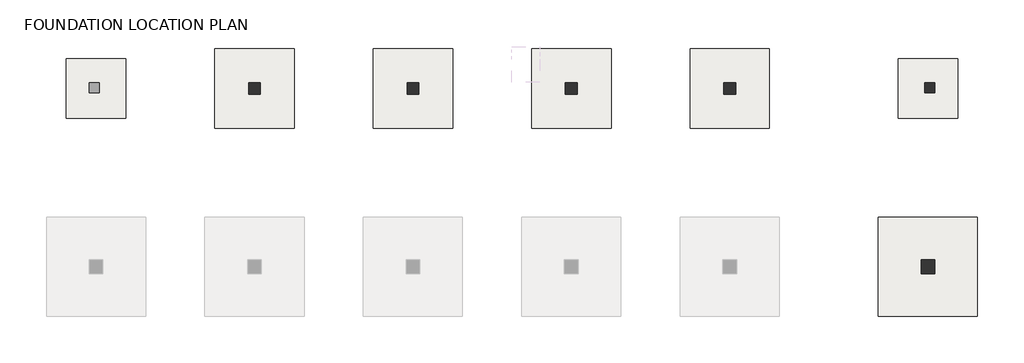
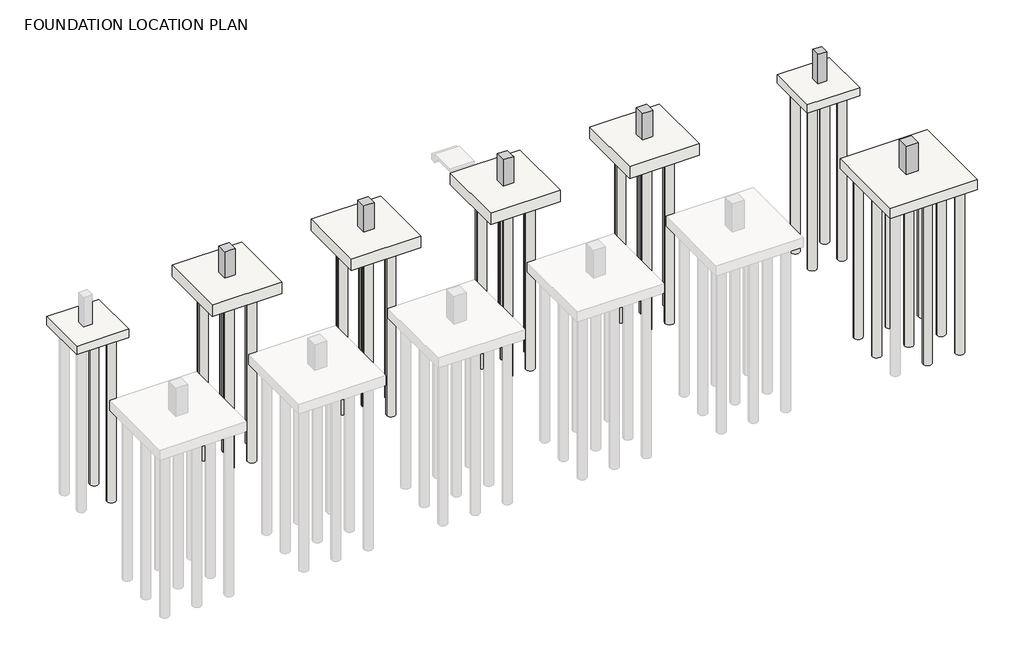
# One storey, part 3 of 3: 49 slabs, 6 columns.
"""IFC4 building model written with IfcOpenShell, lengths in millimetres."""

from ifc_helpers import new_model, si_unit, point, frame, frame_2d, origin, place, context, project, spatial, polyline, circle_curve, trimmed, segment, composite_curve, outline, extrude, faceted_brep, element, save

model = new_model("IFC4")

# Units and contexts
model_context = context("Model", 3, world=origin())
ifc_project = project(units=[si_unit("LENGTHUNIT", "METRE", prefix="MILLI")], contexts=[model_context])

# Site, building, storey
site = spatial("IfcSite", under=ifc_project)
building = spatial("IfcBuilding", under=site)
storey = spatial("IfcBuildingStorey", under=building, Name="FOUNDATION LOCATION PLAN", Elevation=-1699.994759)

# Columns
placement = place(None, origin())
element("IfcColumn", 1, ObjectType="Concrete-Rectangular-Column_R1 : CLS111_RC COLUMN_UG_C1", at=placement, inside=storey, context=model_context, shape_type="Brep", body=[
    faceted_brep([(41850.0, 39299.5208589, -1199.994759), (42350.0, 39299.5208589, -1199.994759), (42350.0, 38799.5208589, -1199.994759), (41850.0, 38799.5208589, -1199.994759), (41850.0, 39299.5208589, 600.005241), (42350.0, 39299.5208589, 600.005241), (41850.0, 38799.5208589, 450.005241), (41850.0, 38799.5208589, 600.005241), (41850.0, 38999.7368538, 600.005241), (42350.0, 38799.5208589, 600.005241), (42000.0, 38799.5208589, 600.005241)], [[[0, 1, 2, 3]], [[1, 0, 4, 5]], [[0, 3, 6, 7, 8, 4]], [[3, 2, 9, 10, 7, 6]], [[2, 1, 5, 9]], [[5, 4, 8, 7, 10, 9]]]),
])
element("IfcColumn", 2, ObjectType="Concrete-Rectangular-Column_R1 : CLS111_RC COLUMN_UG_C3", at=placement, inside=storey, context=model_context, shape_type="Brep", body=[
    faceted_brep([(41650.0, 30349.5208589, -1099.994759), (42350.0, 30349.5208589, -1099.994759), (42350.0, 29649.5208589, -1099.994759), (41650.0, 29649.5208589, -1099.994759), (41650.0, 30349.5208589, 450.005241), (41650.0, 30349.5208589, 600.005241), (42000.0, 30349.5208589, 600.005241), (42350.0, 30349.5208589, 600.005241), (41650.0, 29649.5208589, 450.005241), (41650.0, 29649.5208589, 600.005241), (42350.0, 29649.5208589, 600.005241)], [[[0, 1, 2, 3]], [[1, 0, 4, 5, 6, 7]], [[0, 3, 8, 9, 5, 4]], [[3, 2, 10, 9, 8]], [[2, 1, 7, 10]], [[5, 9, 10, 7, 6]]]),
])
element("IfcColumn", 3, ObjectType="Concrete-Rectangular-Column_R1 : CLS111_RC COLUMN_UG_C2", at=placement, inside=storey, context=model_context, shape_type="Brep", body=[
    faceted_brep([(7700.0, 39299.7368538, -999.994759), (8300.0, 39299.7368538, -999.994759), (8300.0, 38699.7368538, -999.994759), (7700.0, 38699.7368538, -999.994759), (7700.0, 39299.7368538, 600.005241), (8300.0, 39299.7368538, 600.005241), (8300.0, 39299.5208589, 600.005241), (8300.0, 38999.7634659, 600.005241), (8300.0, 38699.7368538, 600.005241), (8300.0, 38699.7368538, 450.005241), (8100.0, 38699.7368538, 600.005241), (7700.0, 38699.7368538, 600.005241), (7700.0, 38699.7368538, 450.005241), (7700.0, 38699.7368538, 0.005241), (7700.0, 38999.7368538, 600.005241), (7700.0, 39299.5208589, 600.005241)], [[[0, 1, 2, 3]], [[1, 0, 4, 5]], [[2, 1, 5, 6, 7, 8, 9]], [[3, 2, 9, 8, 10, 11, 12, 13]], [[0, 3, 13, 12, 11, 14, 15, 4]], [[5, 4, 15, 14, 11, 10, 8, 7, 6]]]),
])
element("IfcColumn", 4, ObjectType="Concrete-Rectangular-Column_R1 : CLS111_RC COLUMN_UG_C2", at=placement, inside=storey, context=model_context, shape_type="Brep", body=[
    faceted_brep([(15700.0, 39299.7368538, -999.994759), (16300.0, 39299.7368538, -999.994759), (16300.0, 38699.7368538, -999.994759), (15700.0, 38699.7368538, -999.994759), (15700.0, 39299.7368538, 600.005241), (16300.0, 39299.7368538, 600.005241), (16300.0, 39299.5208589, 600.005241), (16300.0, 38999.7368538, 600.005241), (16300.0, 38699.7368538, 600.005241), (16300.0, 38699.7368538, 450.005241), (16200.0, 38699.7368538, 600.005241), (15800.0, 38699.7368538, 600.005241), (15700.0, 38699.7368538, 600.005241), (15700.0, 38699.7368538, 450.005241), (15700.0, 38999.7634659, 600.005241), (15700.0, 39299.5208589, 600.005241)], [[[0, 1, 2, 3]], [[1, 0, 4, 5]], [[2, 1, 5, 6, 7, 8, 9]], [[3, 2, 9, 8, 10, 11, 12, 13]], [[0, 3, 13, 12, 14, 15, 4]], [[5, 4, 15, 14, 12, 11, 10, 8, 7, 6]]]),
])
element("IfcColumn", 5, ObjectType="Concrete-Rectangular-Column_R1 : CLS111_RC COLUMN_UG_C2", at=placement, inside=storey, context=model_context, shape_type="Brep", body=[
    faceted_brep([(23700.0, 39299.7368538, -999.994759), (24300.0, 39299.7368538, -999.994759), (24300.0, 38699.7368538, -999.994759), (23700.0, 38699.7368538, -999.994759), (23700.0, 39299.7368538, 600.005241), (24300.0, 39299.7368538, 600.005241), (24300.0, 39299.5208589, 600.005241), (24300.0, 38999.7368538, 600.005241), (24300.0, 38699.7368538, 600.005241), (24300.0, 38699.7368538, 450.005241), (24200.0, 38699.7368538, 600.005241), (23800.0, 38699.7368538, 600.005241), (23700.0, 38699.7368538, 600.005241), (23700.0, 38699.7368538, 450.005241), (23700.0, 38999.7368538, 600.005241), (23700.0, 39299.5208589, 600.005241)], [[[0, 1, 2, 3]], [[1, 0, 4, 5]], [[2, 1, 5, 6, 7, 8, 9]], [[3, 2, 9, 8, 10, 11, 12, 13]], [[0, 3, 13, 12, 14, 15, 4]], [[5, 4, 15, 14, 12, 11, 10, 8, 7, 6]]]),
])
element("IfcColumn", 6, ObjectType="Concrete-Rectangular-Column_R1 : CLS111_RC COLUMN_UG_C2", at=placement, inside=storey, context=model_context, shape_type="Brep", body=[
    faceted_brep([(31700.0, 39299.7368538, -999.994759), (32300.0, 39299.7368538, -999.994759), (32300.0, 38699.7368538, -999.994759), (31700.0, 38699.7368538, -999.994759), (31700.0, 39299.7368538, 600.005241), (32300.0, 39299.7368538, 600.005241), (32300.0, 39299.5208589, 600.005241), (32300.0, 38999.7368538, 600.005241), (32300.0, 38699.7368538, 600.005241), (32300.0, 38699.7368538, 450.005241), (32200.0, 38699.7368538, 600.005241), (31800.0, 38699.7368538, 600.005241), (31700.0, 38699.7368538, 600.005241), (31700.0, 38699.7368538, 450.005241), (31700.0, 38999.7368538, 600.005241), (31700.0, 39299.5208589, 600.005241)], [[[0, 1, 2, 3]], [[1, 0, 4, 5]], [[2, 1, 5, 6, 7, 8, 9]], [[3, 2, 9, 8, 10, 11, 12, 13]], [[0, 3, 13, 12, 14, 15, 4]], [[5, 4, 15, 14, 12, 11, 10, 8, 7, 6]]]),
])

# Slabs
element("IfcSlab", 7, ObjectType="Footing-Rectangular_R1 : FTS301_Footing-Rectangular_3000x3000x500_F1", at=placement, inside=storey, context=model_context, shape_type="SweptSolid", body=[
    extrude(outline(polyline([(1500.0, 40499.7368538), (1500.0, 37499.7368538), (-1500.0, 37499.7368538), (-1500.0, 40499.7368538), (1500.0, 40499.7368538)])), frame((0.0, 0.0, -1699.994759), z_axis=(0.0, 0.0, 1.0), x_axis=(1.0, 0.0, 0.0)), (0.0, 0.0, 1.0), 500.0),
])
element("IfcSlab", 8, ObjectType="Footing-Rectangular_R1 : FTS301_Footing-Rectangular_3000x3000x500_F1", at=placement, inside=storey, context=model_context, shape_type="SweptSolid", body=[
    extrude(outline(polyline([(43500.0, 40499.7368538), (43500.0, 37499.7368538), (40500.0, 37499.7368538), (40500.0, 40499.7368538), (43500.0, 40499.7368538)])), frame((0.0, 0.0, -1699.994759), z_axis=(0.0, 0.0, 1.0), x_axis=(1.0, 0.0, 0.0)), (0.0, 0.0, 1.0), 500.0),
])
element("IfcSlab", 9, ObjectType="Footing-Rectangular_R1 : FTS301_Footing-Rectangular_4000x4000x700_F2", at=placement, inside=storey, context=model_context, shape_type="SweptSolid", body=[
    extrude(outline(polyline([(10000.0, 40999.7368538), (10000.0, 36999.7368538), (6000.0, 36999.7368538), (6000.0, 40999.7368538), (10000.0, 40999.7368538)])), frame((0.0, 0.0, -1699.994759), z_axis=(0.0, 0.0, 1.0), x_axis=(1.0, 0.0, 0.0)), (0.0, 0.0, 1.0), 700.0),
])
element("IfcSlab", 10, ObjectType="Footing-Rectangular_R1 : FTS301_Footing-Rectangular_4000x4000x700_F2", at=placement, inside=storey, context=model_context, shape_type="SweptSolid", body=[
    extrude(outline(polyline([(18000.0, 40999.7368538), (18000.0, 36999.7368538), (14000.0, 36999.7368538), (14000.0, 40999.7368538), (18000.0, 40999.7368538)])), frame((0.0, 0.0, -1699.994759), z_axis=(0.0, 0.0, 1.0), x_axis=(1.0, 0.0, 0.0)), (0.0, 0.0, 1.0), 700.0),
])
element("IfcSlab", 11, ObjectType="Footing-Rectangular_R1 : FTS301_Footing-Rectangular_4000x4000x700_F2", at=placement, inside=storey, context=model_context, shape_type="SweptSolid", body=[
    extrude(outline(polyline([(26000.0, 40999.7368538), (26000.0, 36999.7368538), (22000.0, 36999.7368538), (22000.0, 40999.7368538), (26000.0, 40999.7368538)])), frame((0.0, 0.0, -1699.994759), z_axis=(0.0, 0.0, 1.0), x_axis=(1.0, 0.0, 0.0)), (0.0, 0.0, 1.0), 700.0),
])
element("IfcSlab", 12, ObjectType="Footing-Rectangular_R1 : FTS301_Footing-Rectangular_4000x4000x700_F2", at=placement, inside=storey, context=model_context, shape_type="SweptSolid", body=[
    extrude(outline(polyline([(34000.0, 40999.7368538), (34000.0, 36999.7368538), (30000.0, 36999.7368538), (30000.0, 40999.7368538), (34000.0, 40999.7368538)])), frame((0.0, 0.0, -1699.994759), z_axis=(0.0, 0.0, 1.0), x_axis=(1.0, 0.0, 0.0)), (0.0, 0.0, 1.0), 700.0),
])
element("IfcSlab", 13, ObjectType="Footing-Rectangular_R1 : FTS301_Footing-Rectangular_5000x5000x600_F3", at=placement, inside=storey, context=model_context, shape_type="SweptSolid", body=[
    extrude(outline(polyline([(44500.0, 32499.5208589), (44500.0, 27499.5208589), (39500.0, 27499.5208589), (39500.0, 32499.5208589), (44500.0, 32499.5208589)])), frame((0.0, 0.0, -1699.994759), z_axis=(0.0, 0.0, 1.0), x_axis=(1.0, 0.0, 0.0)), (0.0, 0.0, 1.0), 600.0),
])
element("IfcSlab", 14, ObjectType="HEC_PILE : FTPS102_D500", at=placement, inside=storey, context=model_context, shape_type="SweptSolid", body=[
    extrude(outline(composite_curve([segment(trimmed(circle_curve(frame_2d((850.0, 39849.5208589)), 250.0), [point((600.0, 39849.5208589))], [point((1100.0, 39849.5208589))], False, "CARTESIAN"), True, "CONTINUOUS"), segment(trimmed(circle_curve(frame_2d((850.0, 39849.5208589)), 250.0), [point((1100.0, 39849.5208589))], [point((600.0, 39849.5208589))], False, "CARTESIAN"), True, "CONTINUOUS")], self_intersect=False)), frame((0.0, 0.0, -11749.994759), z_axis=(0.0, 0.0, 1.0), x_axis=(1.0, 0.0, 0.0)), (0.0, 0.0, 1.0), 10150.0),
])
element("IfcSlab", 15, ObjectType="HEC_PILE : FTPS102_D500", at=placement, inside=storey, context=model_context, shape_type="SweptSolid", body=[
    extrude(outline(composite_curve([segment(trimmed(circle_curve(frame_2d((41150.0, 39849.5208589)), 250.0), [point((41400.0, 39849.5208589))], [point((40900.0, 39849.5208589))], False, "CARTESIAN"), True, "CONTINUOUS"), segment(trimmed(circle_curve(frame_2d((41150.0, 39849.5208589)), 250.0), [point((40900.0, 39849.5208589))], [point((41400.0, 39849.5208589))], False, "CARTESIAN"), True, "CONTINUOUS")], self_intersect=False)), frame((0.0, 0.0, -11749.994759), z_axis=(0.0, 0.0, 1.0), x_axis=(1.0, 0.0, 0.0)), (0.0, 0.0, 1.0), 10150.0),
])
element("IfcSlab", 16, ObjectType="HEC_PILE : FTPS102_D500", at=placement, inside=storey, context=model_context, shape_type="SweptSolid", body=[
    extrude(outline(composite_curve([segment(trimmed(circle_curve(frame_2d((42850.0, 39849.5208589)), 250.0), [point((42600.0, 39849.5208589))], [point((43100.0, 39849.5208589))], False, "CARTESIAN"), True, "CONTINUOUS"), segment(trimmed(circle_curve(frame_2d((42850.0, 39849.5208589)), 250.0), [point((43100.0, 39849.5208589))], [point((42600.0, 39849.5208589))], False, "CARTESIAN"), True, "CONTINUOUS")], self_intersect=False)), frame((0.0, 0.0, -11749.994759), z_axis=(0.0, 0.0, 1.0), x_axis=(1.0, 0.0, 0.0)), (0.0, 0.0, 1.0), 10150.0),
])
element("IfcSlab", 17, ObjectType="HEC_PILE : FTPS102_D500", at=placement, inside=storey, context=model_context, shape_type="SweptSolid", body=[
    extrude(outline(composite_curve([segment(trimmed(circle_curve(frame_2d((41150.0, 38149.5208589)), 250.0), [point((41400.0, 38149.5208589))], [point((40900.0, 38149.5208589))], False, "CARTESIAN"), True, "CONTINUOUS"), segment(trimmed(circle_curve(frame_2d((41150.0, 38149.5208589)), 250.0), [point((40900.0, 38149.5208589))], [point((41400.0, 38149.5208589))], False, "CARTESIAN"), True, "CONTINUOUS")], self_intersect=False)), frame((0.0, 0.0, -11749.994759), z_axis=(0.0, 0.0, 1.0), x_axis=(1.0, 0.0, 0.0)), (0.0, 0.0, 1.0), 10150.0),
])
element("IfcSlab", 18, ObjectType="HEC_PILE : FTPS102_D500", at=placement, inside=storey, context=model_context, shape_type="SweptSolid", body=[
    extrude(outline(composite_curve([segment(trimmed(circle_curve(frame_2d((42850.0, 38149.5208589)), 250.0), [point((42600.0, 38149.5208589))], [point((43100.0, 38149.5208589))], False, "CARTESIAN"), True, "CONTINUOUS"), segment(trimmed(circle_curve(frame_2d((42850.0, 38149.5208589)), 250.0), [point((43100.0, 38149.5208589))], [point((42600.0, 38149.5208589))], False, "CARTESIAN"), True, "CONTINUOUS")], self_intersect=False)), frame((0.0, 0.0, -11749.994759), z_axis=(0.0, 0.0, 1.0), x_axis=(1.0, 0.0, 0.0)), (0.0, 0.0, 1.0), 10150.0),
])
element("IfcSlab", 19, ObjectType="HEC_PILE : FTPS102_D500", at=placement, inside=storey, context=model_context, shape_type="SweptSolid", body=[
    extrude(outline(composite_curve([segment(trimmed(circle_curve(frame_2d((31350.0, 37649.5208589)), 250.0), [point((31600.0, 37649.5208589))], [point((31100.0, 37649.5208589))], False, "CARTESIAN"), True, "CONTINUOUS"), segment(trimmed(circle_curve(frame_2d((31350.0, 37649.5208589)), 250.0), [point((31100.0, 37649.5208589))], [point((31600.0, 37649.5208589))], False, "CARTESIAN"), True, "CONTINUOUS")], self_intersect=False)), frame((0.0, 0.0, -11749.994759), z_axis=(0.0, 0.0, 1.0), x_axis=(1.0, 0.0, 0.0)), (0.0, 0.0, 1.0), 10150.0),
])
element("IfcSlab", 20, ObjectType="HEC_PILE : FTPS102_D500", at=placement, inside=storey, context=model_context, shape_type="SweptSolid", body=[
    extrude(outline(composite_curve([segment(trimmed(circle_curve(frame_2d((32650.0, 37649.5208589)), 250.0), [point((32400.0, 37649.5208589))], [point((32900.0, 37649.5208589))], False, "CARTESIAN"), True, "CONTINUOUS"), segment(trimmed(circle_curve(frame_2d((32650.0, 37649.5208589)), 250.0), [point((32900.0, 37649.5208589))], [point((32400.0, 37649.5208589))], False, "CARTESIAN"), True, "CONTINUOUS")], self_intersect=False)), frame((0.0, 0.0, -11749.994759), z_axis=(0.0, 0.0, 1.0), x_axis=(1.0, 0.0, 0.0)), (0.0, 0.0, 1.0), 10150.0),
])
element("IfcSlab", 21, ObjectType="HEC_PILE : FTPS102_D500", at=placement, inside=storey, context=model_context, shape_type="SweptSolid", body=[
    extrude(outline(composite_curve([segment(trimmed(circle_curve(frame_2d((30650.0, 38999.5208589)), 250.0), [point((30900.0, 38999.5208589))], [point((30400.0, 38999.5208589))], False, "CARTESIAN"), True, "CONTINUOUS"), segment(trimmed(circle_curve(frame_2d((30650.0, 38999.5208589)), 250.0), [point((30400.0, 38999.5208589))], [point((30900.0, 38999.5208589))], False, "CARTESIAN"), True, "CONTINUOUS")], self_intersect=False)), frame((0.0, 0.0, -11749.994759), z_axis=(0.0, 0.0, 1.0), x_axis=(1.0, 0.0, 0.0)), (0.0, 0.0, 1.0), 10150.0),
])
element("IfcSlab", 22, ObjectType="HEC_PILE : FTPS102_D500", at=placement, inside=storey, context=model_context, shape_type="SweptSolid", body=[
    extrude(outline(composite_curve([segment(trimmed(circle_curve(frame_2d((32000.0, 38999.5208589)), 250.0), [point((32250.0, 38999.5208589))], [point((31750.0, 38999.5208589))], False, "CARTESIAN"), True, "CONTINUOUS"), segment(trimmed(circle_curve(frame_2d((32000.0, 38999.5208589)), 250.0), [point((31750.0, 38999.5208589))], [point((32250.0, 38999.5208589))], False, "CARTESIAN"), True, "CONTINUOUS")], self_intersect=False)), frame((0.0, 0.0, -11749.994759), z_axis=(0.0, 0.0, 1.0), x_axis=(1.0, 0.0, 0.0)), (0.0, 0.0, 1.0), 10150.0),
])
element("IfcSlab", 23, ObjectType="HEC_PILE : FTPS102_D500", at=placement, inside=storey, context=model_context, shape_type="SweptSolid", body=[
    extrude(outline(composite_curve([segment(trimmed(circle_curve(frame_2d((33350.0, 38999.5208589)), 250.0), [point((33100.0, 38999.5208589))], [point((33600.0, 38999.5208589))], False, "CARTESIAN"), True, "CONTINUOUS"), segment(trimmed(circle_curve(frame_2d((33350.0, 38999.5208589)), 250.0), [point((33600.0, 38999.5208589))], [point((33100.0, 38999.5208589))], False, "CARTESIAN"), True, "CONTINUOUS")], self_intersect=False)), frame((0.0, 0.0, -11749.994759), z_axis=(0.0, 0.0, 1.0), x_axis=(1.0, 0.0, 0.0)), (0.0, 0.0, 1.0), 10150.0),
])
element("IfcSlab", 24, ObjectType="HEC_PILE : FTPS102_D500", at=placement, inside=storey, context=model_context, shape_type="SweptSolid", body=[
    extrude(outline(composite_curve([segment(trimmed(circle_curve(frame_2d((31350.0, 40349.5208589)), 250.0), [point((31600.0, 40349.5208589))], [point((31100.0, 40349.5208589))], False, "CARTESIAN"), True, "CONTINUOUS"), segment(trimmed(circle_curve(frame_2d((31350.0, 40349.5208589)), 250.0), [point((31100.0, 40349.5208589))], [point((31600.0, 40349.5208589))], False, "CARTESIAN"), True, "CONTINUOUS")], self_intersect=False)), frame((0.0, 0.0, -11749.994759), z_axis=(0.0, 0.0, 1.0), x_axis=(1.0, 0.0, 0.0)), (0.0, 0.0, 1.0), 10150.0),
])
element("IfcSlab", 25, ObjectType="HEC_PILE : FTPS102_D500", at=placement, inside=storey, context=model_context, shape_type="SweptSolid", body=[
    extrude(outline(composite_curve([segment(trimmed(circle_curve(frame_2d((32650.0, 40349.5208589)), 250.0), [point((32400.0, 40349.5208589))], [point((32900.0, 40349.5208589))], False, "CARTESIAN"), True, "CONTINUOUS"), segment(trimmed(circle_curve(frame_2d((32650.0, 40349.5208589)), 250.0), [point((32900.0, 40349.5208589))], [point((32400.0, 40349.5208589))], False, "CARTESIAN"), True, "CONTINUOUS")], self_intersect=False)), frame((0.0, 0.0, -11749.994759), z_axis=(0.0, 0.0, 1.0), x_axis=(1.0, 0.0, 0.0)), (0.0, 0.0, 1.0), 10150.0),
])
element("IfcSlab", 26, ObjectType="HEC_PILE : FTPS102_D500", at=placement, inside=storey, context=model_context, shape_type="SweptSolid", body=[
    extrude(outline(composite_curve([segment(trimmed(circle_curve(frame_2d((23350.0, 37649.5208589)), 250.0), [point((23600.0, 37649.5208589))], [point((23100.0, 37649.5208589))], False, "CARTESIAN"), True, "CONTINUOUS"), segment(trimmed(circle_curve(frame_2d((23350.0, 37649.5208589)), 250.0), [point((23100.0, 37649.5208589))], [point((23600.0, 37649.5208589))], False, "CARTESIAN"), True, "CONTINUOUS")], self_intersect=False)), frame((0.0, 0.0, -11749.994759), z_axis=(0.0, 0.0, 1.0), x_axis=(1.0, 0.0, 0.0)), (0.0, 0.0, 1.0), 10150.0),
])
element("IfcSlab", 27, ObjectType="HEC_PILE : FTPS102_D500", at=placement, inside=storey, context=model_context, shape_type="SweptSolid", body=[
    extrude(outline(composite_curve([segment(trimmed(circle_curve(frame_2d((24650.0, 37649.5208589)), 250.0), [point((24400.0, 37649.5208589))], [point((24900.0, 37649.5208589))], False, "CARTESIAN"), True, "CONTINUOUS"), segment(trimmed(circle_curve(frame_2d((24650.0, 37649.5208589)), 250.0), [point((24900.0, 37649.5208589))], [point((24400.0, 37649.5208589))], False, "CARTESIAN"), True, "CONTINUOUS")], self_intersect=False)), frame((0.0, 0.0, -11749.994759), z_axis=(0.0, 0.0, 1.0), x_axis=(1.0, 0.0, 0.0)), (0.0, 0.0, 1.0), 10150.0),
])
element("IfcSlab", 28, ObjectType="HEC_PILE : FTPS102_D500", at=placement, inside=storey, context=model_context, shape_type="SweptSolid", body=[
    extrude(outline(composite_curve([segment(trimmed(circle_curve(frame_2d((22650.0, 38999.5208589)), 250.0), [point((22900.0, 38999.5208589))], [point((22400.0, 38999.5208589))], False, "CARTESIAN"), True, "CONTINUOUS"), segment(trimmed(circle_curve(frame_2d((22650.0, 38999.5208589)), 250.0), [point((22400.0, 38999.5208589))], [point((22900.0, 38999.5208589))], False, "CARTESIAN"), True, "CONTINUOUS")], self_intersect=False)), frame((0.0, 0.0, -11749.994759), z_axis=(0.0, 0.0, 1.0), x_axis=(1.0, 0.0, 0.0)), (0.0, 0.0, 1.0), 10150.0),
])
element("IfcSlab", 29, ObjectType="HEC_PILE : FTPS102_D500", at=placement, inside=storey, context=model_context, shape_type="SweptSolid", body=[
    extrude(outline(composite_curve([segment(trimmed(circle_curve(frame_2d((24000.0, 38999.5208589)), 250.0), [point((24250.0, 38999.5208589))], [point((23750.0, 38999.5208589))], False, "CARTESIAN"), True, "CONTINUOUS"), segment(trimmed(circle_curve(frame_2d((24000.0, 38999.5208589)), 250.0), [point((23750.0, 38999.5208589))], [point((24250.0, 38999.5208589))], False, "CARTESIAN"), True, "CONTINUOUS")], self_intersect=False)), frame((0.0, 0.0, -11749.994759), z_axis=(0.0, 0.0, 1.0), x_axis=(1.0, 0.0, 0.0)), (0.0, 0.0, 1.0), 10150.0),
])
element("IfcSlab", 30, ObjectType="HEC_PILE : FTPS102_D500", at=placement, inside=storey, context=model_context, shape_type="SweptSolid", body=[
    extrude(outline(composite_curve([segment(trimmed(circle_curve(frame_2d((25350.0, 38999.5208589)), 250.0), [point((25100.0, 38999.5208589))], [point((25600.0, 38999.5208589))], False, "CARTESIAN"), True, "CONTINUOUS"), segment(trimmed(circle_curve(frame_2d((25350.0, 38999.5208589)), 250.0), [point((25600.0, 38999.5208589))], [point((25100.0, 38999.5208589))], False, "CARTESIAN"), True, "CONTINUOUS")], self_intersect=False)), frame((0.0, 0.0, -11749.994759), z_axis=(0.0, 0.0, 1.0), x_axis=(1.0, 0.0, 0.0)), (0.0, 0.0, 1.0), 10150.0),
])
element("IfcSlab", 31, ObjectType="HEC_PILE : FTPS102_D500", at=placement, inside=storey, context=model_context, shape_type="SweptSolid", body=[
    extrude(outline(composite_curve([segment(trimmed(circle_curve(frame_2d((23350.0, 40349.5208589)), 250.0), [point((23600.0, 40349.5208589))], [point((23100.0, 40349.5208589))], False, "CARTESIAN"), True, "CONTINUOUS"), segment(trimmed(circle_curve(frame_2d((23350.0, 40349.5208589)), 250.0), [point((23100.0, 40349.5208589))], [point((23600.0, 40349.5208589))], False, "CARTESIAN"), True, "CONTINUOUS")], self_intersect=False)), frame((0.0, 0.0, -11749.994759), z_axis=(0.0, 0.0, 1.0), x_axis=(1.0, 0.0, 0.0)), (0.0, 0.0, 1.0), 10150.0),
])
element("IfcSlab", 32, ObjectType="HEC_PILE : FTPS102_D500", at=placement, inside=storey, context=model_context, shape_type="SweptSolid", body=[
    extrude(outline(composite_curve([segment(trimmed(circle_curve(frame_2d((24650.0, 40349.5208589)), 250.0), [point((24400.0, 40349.5208589))], [point((24900.0, 40349.5208589))], False, "CARTESIAN"), True, "CONTINUOUS"), segment(trimmed(circle_curve(frame_2d((24650.0, 40349.5208589)), 250.0), [point((24900.0, 40349.5208589))], [point((24400.0, 40349.5208589))], False, "CARTESIAN"), True, "CONTINUOUS")], self_intersect=False)), frame((0.0, 0.0, -11749.994759), z_axis=(0.0, 0.0, 1.0), x_axis=(1.0, 0.0, 0.0)), (0.0, 0.0, 1.0), 10150.0),
])
element("IfcSlab", 33, ObjectType="HEC_PILE : FTPS102_D500", at=placement, inside=storey, context=model_context, shape_type="SweptSolid", body=[
    extrude(outline(composite_curve([segment(trimmed(circle_curve(frame_2d((15350.0, 37649.5208589)), 250.0), [point((15600.0, 37649.5208589))], [point((15100.0, 37649.5208589))], False, "CARTESIAN"), True, "CONTINUOUS"), segment(trimmed(circle_curve(frame_2d((15350.0, 37649.5208589)), 250.0), [point((15100.0, 37649.5208589))], [point((15600.0, 37649.5208589))], False, "CARTESIAN"), True, "CONTINUOUS")], self_intersect=False)), frame((0.0, 0.0, -11749.994759), z_axis=(0.0, 0.0, 1.0), x_axis=(1.0, 0.0, 0.0)), (0.0, 0.0, 1.0), 10150.0),
])
element("IfcSlab", 34, ObjectType="HEC_PILE : FTPS102_D500", at=placement, inside=storey, context=model_context, shape_type="SweptSolid", body=[
    extrude(outline(composite_curve([segment(trimmed(circle_curve(frame_2d((16650.0, 37649.5208589)), 250.0), [point((16400.0, 37649.5208589))], [point((16900.0, 37649.5208589))], False, "CARTESIAN"), True, "CONTINUOUS"), segment(trimmed(circle_curve(frame_2d((16650.0, 37649.5208589)), 250.0), [point((16900.0, 37649.5208589))], [point((16400.0, 37649.5208589))], False, "CARTESIAN"), True, "CONTINUOUS")], self_intersect=False)), frame((0.0, 0.0, -11749.994759), z_axis=(0.0, 0.0, 1.0), x_axis=(1.0, 0.0, 0.0)), (0.0, 0.0, 1.0), 10150.0),
])
element("IfcSlab", 35, ObjectType="HEC_PILE : FTPS102_D500", at=placement, inside=storey, context=model_context, shape_type="SweptSolid", body=[
    extrude(outline(composite_curve([segment(trimmed(circle_curve(frame_2d((14650.0, 38999.5208589)), 250.0), [point((14900.0, 38999.5208589))], [point((14400.0, 38999.5208589))], False, "CARTESIAN"), True, "CONTINUOUS"), segment(trimmed(circle_curve(frame_2d((14650.0, 38999.5208589)), 250.0), [point((14400.0, 38999.5208589))], [point((14900.0, 38999.5208589))], False, "CARTESIAN"), True, "CONTINUOUS")], self_intersect=False)), frame((0.0, 0.0, -11749.994759), z_axis=(0.0, 0.0, 1.0), x_axis=(1.0, 0.0, 0.0)), (0.0, 0.0, 1.0), 10150.0),
])
element("IfcSlab", 36, ObjectType="HEC_PILE : FTPS102_D500", at=placement, inside=storey, context=model_context, shape_type="SweptSolid", body=[
    extrude(outline(composite_curve([segment(trimmed(circle_curve(frame_2d((16000.0, 38999.5208589)), 250.0), [point((16250.0, 38999.5208589))], [point((15750.0, 38999.5208589))], False, "CARTESIAN"), True, "CONTINUOUS"), segment(trimmed(circle_curve(frame_2d((16000.0, 38999.5208589)), 250.0), [point((15750.0, 38999.5208589))], [point((16250.0, 38999.5208589))], False, "CARTESIAN"), True, "CONTINUOUS")], self_intersect=False)), frame((0.0, 0.0, -11749.994759), z_axis=(0.0, 0.0, 1.0), x_axis=(1.0, 0.0, 0.0)), (0.0, 0.0, 1.0), 10150.0),
])
element("IfcSlab", 37, ObjectType="HEC_PILE : FTPS102_D500", at=placement, inside=storey, context=model_context, shape_type="SweptSolid", body=[
    extrude(outline(composite_curve([segment(trimmed(circle_curve(frame_2d((17350.0, 38999.5208589)), 250.0), [point((17100.0, 38999.5208589))], [point((17600.0, 38999.5208589))], False, "CARTESIAN"), True, "CONTINUOUS"), segment(trimmed(circle_curve(frame_2d((17350.0, 38999.5208589)), 250.0), [point((17600.0, 38999.5208589))], [point((17100.0, 38999.5208589))], False, "CARTESIAN"), True, "CONTINUOUS")], self_intersect=False)), frame((0.0, 0.0, -11749.994759), z_axis=(0.0, 0.0, 1.0), x_axis=(1.0, 0.0, 0.0)), (0.0, 0.0, 1.0), 10150.0),
])
element("IfcSlab", 38, ObjectType="HEC_PILE : FTPS102_D500", at=placement, inside=storey, context=model_context, shape_type="SweptSolid", body=[
    extrude(outline(composite_curve([segment(trimmed(circle_curve(frame_2d((15350.0, 40349.5208589)), 250.0), [point((15600.0, 40349.5208589))], [point((15100.0, 40349.5208589))], False, "CARTESIAN"), True, "CONTINUOUS"), segment(trimmed(circle_curve(frame_2d((15350.0, 40349.5208589)), 250.0), [point((15100.0, 40349.5208589))], [point((15600.0, 40349.5208589))], False, "CARTESIAN"), True, "CONTINUOUS")], self_intersect=False)), frame((0.0, 0.0, -11749.994759), z_axis=(0.0, 0.0, 1.0), x_axis=(1.0, 0.0, 0.0)), (0.0, 0.0, 1.0), 10150.0),
])
element("IfcSlab", 39, ObjectType="HEC_PILE : FTPS102_D500", at=placement, inside=storey, context=model_context, shape_type="SweptSolid", body=[
    extrude(outline(composite_curve([segment(trimmed(circle_curve(frame_2d((16650.0, 40349.5208589)), 250.0), [point((16400.0, 40349.5208589))], [point((16900.0, 40349.5208589))], False, "CARTESIAN"), True, "CONTINUOUS"), segment(trimmed(circle_curve(frame_2d((16650.0, 40349.5208589)), 250.0), [point((16900.0, 40349.5208589))], [point((16400.0, 40349.5208589))], False, "CARTESIAN"), True, "CONTINUOUS")], self_intersect=False)), frame((0.0, 0.0, -11749.994759), z_axis=(0.0, 0.0, 1.0), x_axis=(1.0, 0.0, 0.0)), (0.0, 0.0, 1.0), 10150.0),
])
element("IfcSlab", 40, ObjectType="HEC_PILE : FTPS102_D500", at=placement, inside=storey, context=model_context, shape_type="SweptSolid", body=[
    extrude(outline(composite_curve([segment(trimmed(circle_curve(frame_2d((7350.0, 37649.5208589)), 250.0), [point((7600.0, 37649.5208589))], [point((7100.0, 37649.5208589))], False, "CARTESIAN"), True, "CONTINUOUS"), segment(trimmed(circle_curve(frame_2d((7350.0, 37649.5208589)), 250.0), [point((7100.0, 37649.5208589))], [point((7600.0, 37649.5208589))], False, "CARTESIAN"), True, "CONTINUOUS")], self_intersect=False)), frame((0.0, 0.0, -11749.994759), z_axis=(0.0, 0.0, 1.0), x_axis=(1.0, 0.0, 0.0)), (0.0, 0.0, 1.0), 10150.0),
])
element("IfcSlab", 41, ObjectType="HEC_PILE : FTPS102_D500", at=placement, inside=storey, context=model_context, shape_type="SweptSolid", body=[
    extrude(outline(composite_curve([segment(trimmed(circle_curve(frame_2d((8650.0, 37649.5208589)), 250.0), [point((8400.0, 37649.5208589))], [point((8900.0, 37649.5208589))], False, "CARTESIAN"), True, "CONTINUOUS"), segment(trimmed(circle_curve(frame_2d((8650.0, 37649.5208589)), 250.0), [point((8900.0, 37649.5208589))], [point((8400.0, 37649.5208589))], False, "CARTESIAN"), True, "CONTINUOUS")], self_intersect=False)), frame((0.0, 0.0, -11749.994759), z_axis=(0.0, 0.0, 1.0), x_axis=(1.0, 0.0, 0.0)), (0.0, 0.0, 1.0), 10150.0),
])
element("IfcSlab", 42, ObjectType="HEC_PILE : FTPS102_D500", at=placement, inside=storey, context=model_context, shape_type="SweptSolid", body=[
    extrude(outline(composite_curve([segment(trimmed(circle_curve(frame_2d((6650.0, 38999.5208589)), 250.0), [point((6900.0, 38999.5208589))], [point((6400.0, 38999.5208589))], False, "CARTESIAN"), True, "CONTINUOUS"), segment(trimmed(circle_curve(frame_2d((6650.0, 38999.5208589)), 250.0), [point((6400.0, 38999.5208589))], [point((6900.0, 38999.5208589))], False, "CARTESIAN"), True, "CONTINUOUS")], self_intersect=False)), frame((0.0, 0.0, -11749.994759), z_axis=(0.0, 0.0, 1.0), x_axis=(1.0, 0.0, 0.0)), (0.0, 0.0, 1.0), 10150.0),
])
element("IfcSlab", 43, ObjectType="HEC_PILE : FTPS102_D500", at=placement, inside=storey, context=model_context, shape_type="SweptSolid", body=[
    extrude(outline(composite_curve([segment(trimmed(circle_curve(frame_2d((8000.0, 38999.5208589)), 250.0), [point((8250.0, 38999.5208589))], [point((7750.0, 38999.5208589))], False, "CARTESIAN"), True, "CONTINUOUS"), segment(trimmed(circle_curve(frame_2d((8000.0, 38999.5208589)), 250.0), [point((7750.0, 38999.5208589))], [point((8250.0, 38999.5208589))], False, "CARTESIAN"), True, "CONTINUOUS")], self_intersect=False)), frame((0.0, 0.0, -11749.994759), z_axis=(0.0, 0.0, 1.0), x_axis=(1.0, 0.0, 0.0)), (0.0, 0.0, 1.0), 10150.0),
])
element("IfcSlab", 44, ObjectType="HEC_PILE : FTPS102_D500", at=placement, inside=storey, context=model_context, shape_type="SweptSolid", body=[
    extrude(outline(composite_curve([segment(trimmed(circle_curve(frame_2d((9350.0, 38999.5208589)), 250.0), [point((9100.0, 38999.5208589))], [point((9600.0, 38999.5208589))], False, "CARTESIAN"), True, "CONTINUOUS"), segment(trimmed(circle_curve(frame_2d((9350.0, 38999.5208589)), 250.0), [point((9600.0, 38999.5208589))], [point((9100.0, 38999.5208589))], False, "CARTESIAN"), True, "CONTINUOUS")], self_intersect=False)), frame((0.0, 0.0, -11749.994759), z_axis=(0.0, 0.0, 1.0), x_axis=(1.0, 0.0, 0.0)), (0.0, 0.0, 1.0), 10150.0),
])
element("IfcSlab", 45, ObjectType="HEC_PILE : FTPS102_D500", at=placement, inside=storey, context=model_context, shape_type="SweptSolid", body=[
    extrude(outline(composite_curve([segment(trimmed(circle_curve(frame_2d((7350.0, 40349.5208589)), 250.0), [point((7600.0, 40349.5208589))], [point((7100.0, 40349.5208589))], False, "CARTESIAN"), True, "CONTINUOUS"), segment(trimmed(circle_curve(frame_2d((7350.0, 40349.5208589)), 250.0), [point((7100.0, 40349.5208589))], [point((7600.0, 40349.5208589))], False, "CARTESIAN"), True, "CONTINUOUS")], self_intersect=False)), frame((0.0, 0.0, -11749.994759), z_axis=(0.0, 0.0, 1.0), x_axis=(1.0, 0.0, 0.0)), (0.0, 0.0, 1.0), 10150.0),
])
element("IfcSlab", 46, ObjectType="HEC_PILE : FTPS102_D500", at=placement, inside=storey, context=model_context, shape_type="SweptSolid", body=[
    extrude(outline(composite_curve([segment(trimmed(circle_curve(frame_2d((8650.0, 40349.5208589)), 250.0), [point((8400.0, 40349.5208589))], [point((8900.0, 40349.5208589))], False, "CARTESIAN"), True, "CONTINUOUS"), segment(trimmed(circle_curve(frame_2d((8650.0, 40349.5208589)), 250.0), [point((8900.0, 40349.5208589))], [point((8400.0, 40349.5208589))], False, "CARTESIAN"), True, "CONTINUOUS")], self_intersect=False)), frame((0.0, 0.0, -11749.994759), z_axis=(0.0, 0.0, 1.0), x_axis=(1.0, 0.0, 0.0)), (0.0, 0.0, 1.0), 10150.0),
])
element("IfcSlab", 47, ObjectType="HEC_PILE : FTPS102_D500", at=placement, inside=storey, context=model_context, shape_type="SweptSolid", body=[
    extrude(outline(composite_curve([segment(trimmed(circle_curve(frame_2d((40150.0, 29999.5208589)), 250.0), [point((40400.0, 29999.5208589))], [point((39900.0, 29999.5208589))], False, "CARTESIAN"), True, "CONTINUOUS"), segment(trimmed(circle_curve(frame_2d((40150.0, 29999.5208589)), 250.0), [point((39900.0, 29999.5208589))], [point((40400.0, 29999.5208589))], False, "CARTESIAN"), True, "CONTINUOUS")], self_intersect=False)), frame((0.0, 0.0, -11749.994759), z_axis=(0.0, 0.0, 1.0), x_axis=(1.0, 0.0, 0.0)), (0.0, 0.0, 1.0), 10150.0),
])
element("IfcSlab", 48, ObjectType="HEC_PILE : FTPS102_D500", at=placement, inside=storey, context=model_context, shape_type="SweptSolid", body=[
    extrude(outline(composite_curve([segment(trimmed(circle_curve(frame_2d((43850.0, 29999.5208589)), 250.0), [point((43600.0, 29999.5208589))], [point((44100.0, 29999.5208589))], False, "CARTESIAN"), True, "CONTINUOUS"), segment(trimmed(circle_curve(frame_2d((43850.0, 29999.5208589)), 250.0), [point((44100.0, 29999.5208589))], [point((43600.0, 29999.5208589))], False, "CARTESIAN"), True, "CONTINUOUS")], self_intersect=False)), frame((0.0, 0.0, -11749.994759), z_axis=(0.0, 0.0, 1.0), x_axis=(1.0, 0.0, 0.0)), (0.0, 0.0, 1.0), 10150.0),
])
element("IfcSlab", 49, ObjectType="HEC_PILE : FTPS102_D500", at=placement, inside=storey, context=model_context, shape_type="SweptSolid", body=[
    extrude(outline(composite_curve([segment(trimmed(circle_curve(frame_2d((42000.0, 29999.5208589)), 250.0), [point((41750.0, 29999.5208589))], [point((42250.0, 29999.5208589))], False, "CARTESIAN"), True, "CONTINUOUS"), segment(trimmed(circle_curve(frame_2d((42000.0, 29999.5208589)), 250.0), [point((42250.0, 29999.5208589))], [point((41750.0, 29999.5208589))], False, "CARTESIAN"), True, "CONTINUOUS")], self_intersect=False)), frame((0.0, 0.0, -11749.994759), z_axis=(0.0, 0.0, 1.0), x_axis=(1.0, 0.0, 0.0)), (0.0, 0.0, 1.0), 10150.0),
])
element("IfcSlab", 50, ObjectType="HEC_PILE : FTPS102_D500", at=placement, inside=storey, context=model_context, shape_type="SweptSolid", body=[
    extrude(outline(composite_curve([segment(trimmed(circle_curve(frame_2d((40150.0, 31849.5208589)), 250.0), [point((40400.0, 31849.5208589))], [point((39900.0, 31849.5208589))], False, "CARTESIAN"), True, "CONTINUOUS"), segment(trimmed(circle_curve(frame_2d((40150.0, 31849.5208589)), 250.0), [point((39900.0, 31849.5208589))], [point((40400.0, 31849.5208589))], False, "CARTESIAN"), True, "CONTINUOUS")], self_intersect=False)), frame((0.0, 0.0, -11749.994759), z_axis=(0.0, 0.0, 1.0), x_axis=(1.0, 0.0, 0.0)), (0.0, 0.0, 1.0), 10150.0),
])
element("IfcSlab", 51, ObjectType="HEC_PILE : FTPS102_D500", at=placement, inside=storey, context=model_context, shape_type="SweptSolid", body=[
    extrude(outline(composite_curve([segment(trimmed(circle_curve(frame_2d((43850.0, 31849.5208589)), 250.0), [point((43600.0, 31849.5208589))], [point((44100.0, 31849.5208589))], False, "CARTESIAN"), True, "CONTINUOUS"), segment(trimmed(circle_curve(frame_2d((43850.0, 31849.5208589)), 250.0), [point((44100.0, 31849.5208589))], [point((43600.0, 31849.5208589))], False, "CARTESIAN"), True, "CONTINUOUS")], self_intersect=False)), frame((0.0, 0.0, -11749.994759), z_axis=(0.0, 0.0, 1.0), x_axis=(1.0, 0.0, 0.0)), (0.0, 0.0, 1.0), 10150.0),
])
element("IfcSlab", 52, ObjectType="HEC_PILE : FTPS102_D500", at=placement, inside=storey, context=model_context, shape_type="SweptSolid", body=[
    extrude(outline(composite_curve([segment(trimmed(circle_curve(frame_2d((42000.0, 31849.5208589)), 250.0), [point((41750.0, 31849.5208589))], [point((42250.0, 31849.5208589))], False, "CARTESIAN"), True, "CONTINUOUS"), segment(trimmed(circle_curve(frame_2d((42000.0, 31849.5208589)), 250.0), [point((42250.0, 31849.5208589))], [point((41750.0, 31849.5208589))], False, "CARTESIAN"), True, "CONTINUOUS")], self_intersect=False)), frame((0.0, 0.0, -11749.994759), z_axis=(0.0, 0.0, 1.0), x_axis=(1.0, 0.0, 0.0)), (0.0, 0.0, 1.0), 10150.0),
])
element("IfcSlab", 53, ObjectType="HEC_PILE : FTPS102_D500", at=placement, inside=storey, context=model_context, shape_type="SweptSolid", body=[
    extrude(outline(composite_curve([segment(trimmed(circle_curve(frame_2d((43850.0, 28149.5208589)), 250.0), [point((43600.0, 28149.5208589))], [point((44100.0, 28149.5208589))], False, "CARTESIAN"), True, "CONTINUOUS"), segment(trimmed(circle_curve(frame_2d((43850.0, 28149.5208589)), 250.0), [point((44100.0, 28149.5208589))], [point((43600.0, 28149.5208589))], False, "CARTESIAN"), True, "CONTINUOUS")], self_intersect=False)), frame((0.0, 0.0, -11749.994759), z_axis=(0.0, 0.0, 1.0), x_axis=(1.0, 0.0, 0.0)), (0.0, 0.0, 1.0), 10150.0),
])
element("IfcSlab", 54, ObjectType="HEC_PILE : FTPS102_D500", at=placement, inside=storey, context=model_context, shape_type="SweptSolid", body=[
    extrude(outline(composite_curve([segment(trimmed(circle_curve(frame_2d((42000.0, 28149.5208589)), 250.0), [point((41750.0, 28149.5208589))], [point((42250.0, 28149.5208589))], False, "CARTESIAN"), True, "CONTINUOUS"), segment(trimmed(circle_curve(frame_2d((42000.0, 28149.5208589)), 250.0), [point((42250.0, 28149.5208589))], [point((41750.0, 28149.5208589))], False, "CARTESIAN"), True, "CONTINUOUS")], self_intersect=False)), frame((0.0, 0.0, -11749.994759), z_axis=(0.0, 0.0, 1.0), x_axis=(1.0, 0.0, 0.0)), (0.0, 0.0, 1.0), 10150.0),
])
element("IfcSlab", 55, ObjectType="HEC_PILE : FTPS102_D500", at=placement, inside=storey, context=model_context, shape_type="SweptSolid", body=[
    extrude(outline(composite_curve([segment(trimmed(circle_curve(frame_2d((850.0, 38149.9528486)), 250.0), [point((600.0, 38149.9528486))], [point((1100.0, 38149.9528486))], False, "CARTESIAN"), True, "CONTINUOUS"), segment(trimmed(circle_curve(frame_2d((850.0, 38149.9528486)), 250.0), [point((1100.0, 38149.9528486))], [point((600.0, 38149.9528486))], False, "CARTESIAN"), True, "CONTINUOUS")], self_intersect=False)), frame((0.0, 0.0, -11749.994759), z_axis=(0.0, 0.0, 1.0), x_axis=(1.0, 0.0, 0.0)), (0.0, 0.0, 1.0), 10150.0),
])

save(model, "model.ifc")

# Revit data of these elements
# Type "Concrete-Rectangular-Column_R1 : CLS111_RC COLUMN_UG_C1"
#   Description = "AG RC 기둥"
#   Width = 500 mm
#   Length = 500 mm
#   hec_material3 [instance default] = none
#   hec_material2 [instance default] = A03AE056-00001_Bitumen/Bituminous/Asphalt Coating
#   hec_material1 [instance default] = A03AC035-00001_Form Work (3 times in use)_Flat
#   Structural Material [instance default] = A03AC032-00007_Structural Concrete_Type1_25MPa-30Mpa
# Type "Concrete-Rectangular-Column_R1 : CLS111_RC COLUMN_UG_C3"
#   Description = "AG RC 기둥"
#   Width = 700 mm
#   Length = 700 mm
#   hec_material3 [instance default] = none
#   hec_material2 [instance default] = A03AE056-00001_Bitumen/Bituminous/Asphalt Coating
#   hec_material1 [instance default] = A03AC035-00001_Form Work (3 times in use)_Flat
#   Structural Material [instance default] = A03AC032-00007_Structural Concrete_Type1_25MPa-30Mpa
# Type "Concrete-Rectangular-Column_R1 : CLS111_RC COLUMN_UG_C2"
#   Description = "AG RC 기둥"
#   Width = 600 mm
#   Length = 600 mm
#   hec_material3 [instance default] = none
#   hec_material2 [instance default] = A03AE056-00001_Bitumen/Bituminous/Asphalt Coating
#   hec_material1 [instance default] = A03AC035-00001_Form Work (3 times in use)_Flat
#   Structural Material [instance default] = A03AC032-00007_Structural Concrete_Type1_25MPa-30Mpa
# Type "Footing-Rectangular_R1 : FTS301_Footing-Rectangular_3000x3000x500_F1"
#   Type Mark = "F1"
#   Top bar = "D25@300"
#   Description = "UG Shallow Foundation"
#   Bottom bar = "D20@300"
#   Width = 3000 mm
#   Length = 3000 mm
#   Foundation Thickness = 500 mm
#   Structural Material [instance default] = A03AC032-00007_Structural Concrete_Type1_25MPa-30Mpa
#   Assembly Code = ""
# Type "Footing-Rectangular_R1 : FTS301_Footing-Rectangular_4000x4000x700_F2"
#   Type Mark = "F2"
#   Top bar = "D25@300"
#   Description = "UG Shallow Foundation"
#   Bottom bar = "D20@300"
#   Width = 4000 mm
#   Length = 4000 mm
#   Foundation Thickness = 700 mm
#   Structural Material [instance default] = A03AC032-00007_Structural Concrete_Type1_25MPa-30Mpa
#   Assembly Code = ""
# Type "Footing-Rectangular_R1 : FTS301_Footing-Rectangular_5000x5000x600_F3"
#   Type Mark = "F3"
#   Top bar = "D25@300"
#   Description = "UG Shallow Foundation"
#   Bottom bar = "D20@300"
#   Width = 5000 mm
#   Length = 5000 mm
#   Foundation Thickness = 600 mm
#   Structural Material [instance default] = A03AC032-00007_Structural Concrete_Type1_25MPa-30Mpa
#   Assembly Code = ""
# Type "HEC_PILE : FTPS102_D500"
#   Assembly Code = "A1020130"
#   반지름 = 250 mm
#   최소 내포 = 150 mm
#   Diameter = 500 mm
#   Depth = 10000 mm
#   구조 재료 = A02AA014-00001_Piling Work_Reinforced Concrete Pile(Round Type)_Direct Driving
# Element 1 (IfcColumn, "Concrete-Rectangular-Column_R1 : CLS111_RC COLUMN_UG_C1")
#   Mark = "C1"
#   Structural Material = A03AC032-00007_Structural Concrete_Type1_25MPa-30Mpa
#   hec_material3 = none
#   hec_material2 = A03AE056-00001_Bitumen/Bituminous/Asphalt Coating
#   hec_material1 = A03AC035-00001_Form Work (3 times in use)_Flat
#   Phase Created = New Construction
#   Materials on its faces: "A03AC032-00007_Structural Concrete_Type1_25MPa-30Mpa"
# Element 2 (IfcColumn, "Concrete-Rectangular-Column_R1 : CLS111_RC COLUMN_UG_C3")
#   Mark = "C3"
#   Structural Material = A03AC032-00007_Structural Concrete_Type1_25MPa-30Mpa
#   hec_material3 = none
#   hec_material2 = A03AE056-00001_Bitumen/Bituminous/Asphalt Coating
#   hec_material1 = A03AC035-00001_Form Work (3 times in use)_Flat
#   Phase Created = New Construction
#   Materials on its faces: "A03AC032-00007_Structural Concrete_Type1_25MPa-30Mpa"
# Elements 3, 4, 5, 6 (IfcColumn, "Concrete-Rectangular-Column_R1 : CLS111_RC COLUMN_UG_C2")
#   Mark = "C2"
#   Structural Material = A03AC032-00007_Structural Concrete_Type1_25MPa-30Mpa
#   hec_material3 = none
#   hec_material2 = A03AE056-00001_Bitumen/Bituminous/Asphalt Coating
#   hec_material1 = A03AC035-00001_Form Work (3 times in use)_Flat
#   Phase Created = New Construction
#   Materials on its faces: "A03AC032-00007_Structural Concrete_Type1_25MPa-30Mpa"
# Elements 7, 8 (IfcSlab, "Footing-Rectangular_R1 : FTS301_Footing-Rectangular_3000x3000x500_F1")
#   Comments = ""
#   Structural Material = A03AC032-00007_Structural Concrete_Type1_25MPa-30Mpa
#   Phase Created = New Construction
#   Materials on its faces: "A03AC032-00007_Structural Concrete_Type1_25MPa-30Mpa"
# Elements 9, 10, 11, 12 (IfcSlab, "Footing-Rectangular_R1 : FTS301_Footing-Rectangular_4000x4000x700_F2")
#   Comments = ""
#   Structural Material = A03AC032-00007_Structural Concrete_Type1_25MPa-30Mpa
#   Phase Created = New Construction
#   Materials on its faces: "A03AC032-00007_Structural Concrete_Type1_25MPa-30Mpa"
# Element 13 (IfcSlab, "Footing-Rectangular_R1 : FTS301_Footing-Rectangular_5000x5000x600_F3")
#   Comments = ""
#   Structural Material = A03AC032-00007_Structural Concrete_Type1_25MPa-30Mpa
#   Phase Created = New Construction
#   Materials on its faces: "A03AC032-00007_Structural Concrete_Type1_25MPa-30Mpa"
# Elements 14, 15, 16, 17, 18, 19, 20, 21, 22, 23, 24, 25, 26, 27, 28, 29, 30, 31, 32, 33, 34, 35, 36, 37, 38, 39, 40, 41, 42, 43, 44, 45, 46, 47, 48, 49, 50, 51, 52, 53, 54, 55 (IfcSlab, "HEC_PILE : FTPS102_D500")
#   F01) Building Name = "STEAM TURBINE BLDG"
#   Phase Created = New Construction
#   Materials on its faces: "A02AA014-00001_Piling Work_Reinforced Concrete Pile(Round Type)_Direct Driving"
# Materials
#   "A03AE056-00001_Bitumen/Bituminous/Asphalt Coating": class "Generic", colour RGB 17 17 17, transparency 0, Description = "Damp-proofing", W00) Work Master Code = "A03AE056-00001", W01) Work Master_Lv1 = "Concrete Work", W02) Work Master_Lv2 = "Concrete Protective Coating (U/G)", W03) Work Master_Spec.1 = "Bitumen/Bituminous/Asphalt Coating", Cost = 0
#   "A03AC035-00001_Form Work (3 times in use)_Flat": class "Wood", colour RGB 149 120 74, transparency 0, Description = "Plywood", W00) Work Master Code = "A03AC035-00001", W01) Work Master_Lv1 = "Concrete Work", W02) Work Master_Lv2 = "Substructure Work", W03) Work Master_Spec.1 = "Form Work (3 times in use)", W04) Work Master_Spec.2 = "Flat Form", W05) Work Master_Spec.3 = "Dressed Lumber, Plywood or Steel Form(Wood Planks are not Allowed) incl. Chamfer", Cost = 0
#   "A03AC032-00007_Structural Concrete_Type1_25MPa-30Mpa": class "Concrete", colour RGB 176 176 176, transparency 0, Keynote = "09910.A1", Description = "Reinf. Conc.", W00) Work Master Code = "A03AC032-00007", W01) Work Master_Lv1 = "Concrete Work", W02) Work Master_Lv2 = "Substructure Work", W03) Work Master_Spec.1 = "Structural Concrete", W04) Work Master_Spec.2 = "Cement Type-1", W05) Work Master_Spec.3 = "25MPa < F'c (Cylinder Strength) ≤ 30MPa", Cost = 0
#   "A02AA014-00001_Piling Work_Reinforced Concrete Pile(Round Type)_Direct Driving": class "Concrete", colour RGB 176 176 176, transparency 0, Keynote = "09910.A1", Description = "Reinf. Conc.", Cost = 0
